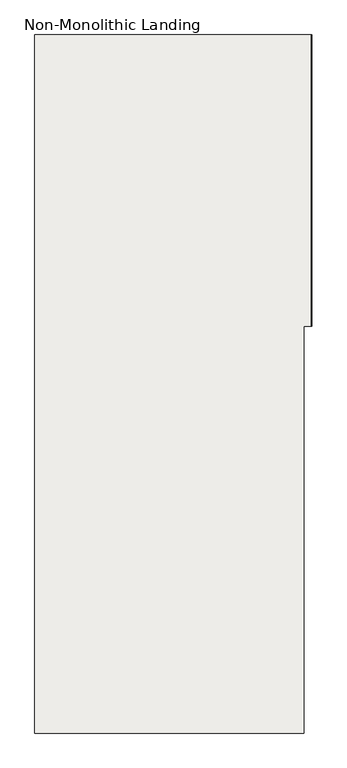
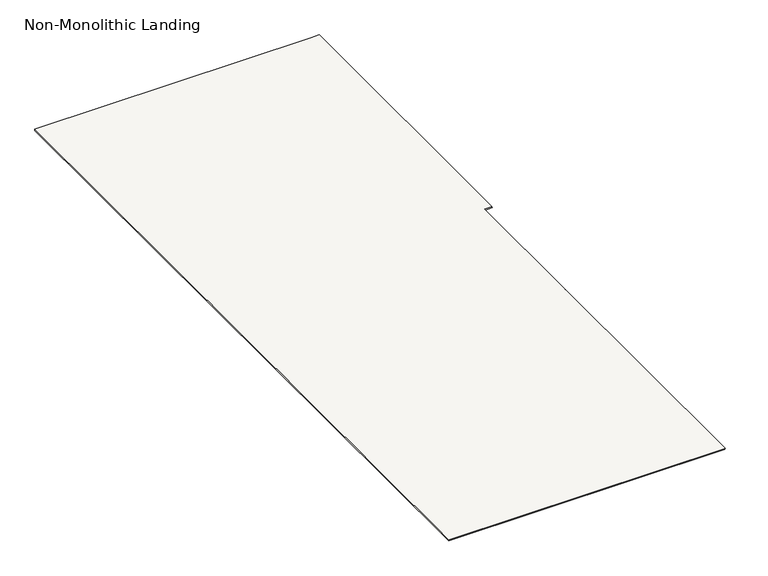
"""IFC4 building model written with IfcOpenShell, lengths in millimetres: slab geometry, Non-Monolithic Landing."""

from ifc_helpers import new_model, si_unit, origin, place, context, project, spatial, faceted_brep, source, transform, mapped, element, save


def non_monolithic_landing_5c894f0a(model_context):
    return source(origin(), model_context, "Body", "Brep", [
        faceted_brep([(-16318.9400908, 12030.4345331, 14176.4705882), (-16318.0900908, 12030.4345331, 14170.4705882), (-16318.0900908, 13220.4345331, 14170.4705882), (-16318.9400908, 13220.4345331, 14176.4705882), (-16350.0, 11470.4345331, 14176.4705882), (-16350.0, 12030.4345331, 14176.4705882), (-16350.0, 13220.4345331, 14176.4705882), (-17450.0, 13220.4345331, 14176.4705882), (-17450.0, 10370.4345331, 14176.4705882), (-16350.0, 10370.4345331, 14176.4705882), (-16350.0, 12030.4345331, 14170.4705882), (-16350.0, 11470.4345331, 14170.4705882), (-16350.85, 11470.4345331, 14170.4705882), (-16350.85, 10370.4345331, 14170.4705882), (-17450.0, 10370.4345331, 14170.4705882), (-17450.0, 13220.4345331, 14170.4705882), (-16350.0, 13220.4345331, 14170.4705882)], [[[0, 1, 2, 3]], [[4, 5, 0, 3, 6, 7, 8, 9]], [[10, 11, 12, 13, 14, 15, 16, 2, 1]], [[5, 4, 11, 10]], [[0, 5, 10, 1]], [[6, 3, 2, 16]], [[7, 6, 16, 15]], [[8, 7, 15, 14]], [[9, 8, 14, 13]], [[4, 12, 11]], [[12, 4, 9, 13]]]),
    ])


if __name__ == "__main__":
    model = new_model("IFC4")
    model_context = context("Model", 3, world=origin())
    ifc_project = project(units=[si_unit("LENGTHUNIT", "METRE", prefix="MILLI")], contexts=[model_context])
    site = spatial("IfcSite", under=ifc_project)
    building = spatial("IfcBuilding", under=site)
    placement = place(None, origin())
    non_monolithic_landing_shape = non_monolithic_landing_5c894f0a(model_context)
    element("IfcSlab", 1, ObjectType="Non-Monolithic Landing", at=placement, inside=building, context=model_context, shape_type="MappedRepresentation", body=[
        mapped(non_monolithic_landing_shape, transform((0.0, 0.0, 0.0), x_axis=(1.0, 0.0, 0.0), y_axis=(0.0, 1.0, 0.0), z_axis=(0.0, 0.0, 1.0))),
    ])
    save(model, "model.ifc")

# Revit data of these elements
# Element 1 (IfcSlab, "Non-Monolithic Landing")
#   Materials on its faces: "Steel, Paint Finish, Dark Gray"
# Materials
#   "Steel, Paint Finish, Dark Gray": class "Metal", colour RGB 89 89 89, transparency 0, Description = "Steel, paint finish, dark gray, glossy", Cost = 0
